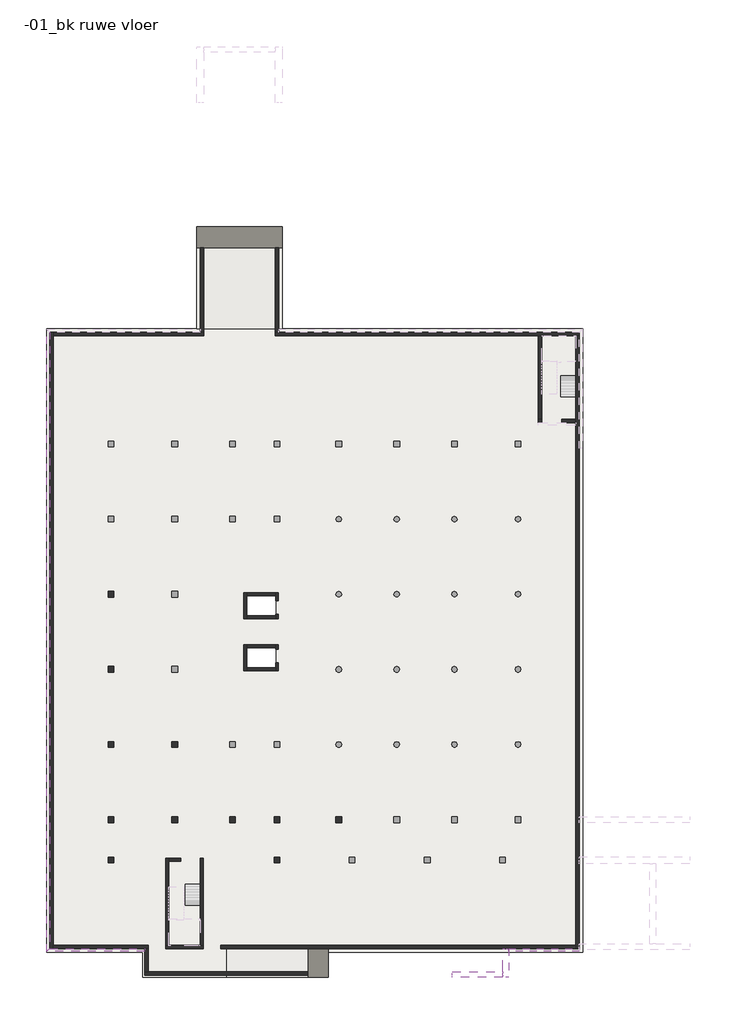
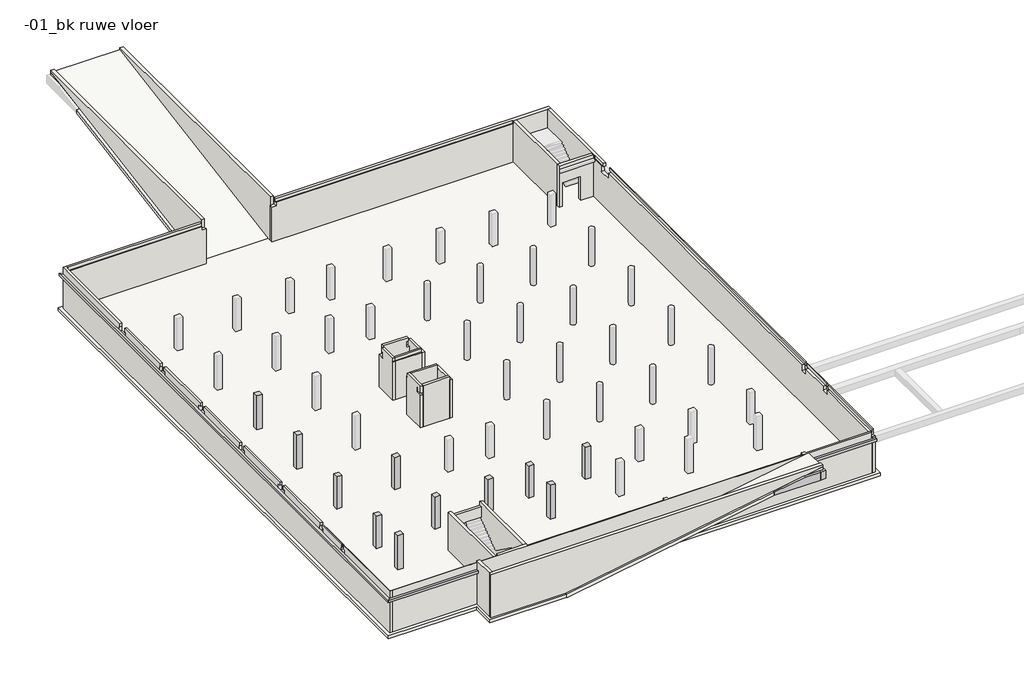
# One storey, part 1 of 2: 22 walls, 15 slabs, 11 columns, 5 beams.
# Revit data of these elements (continued)
# Grids (mm) (continued)
#   "L": line (13000, -4030.51) -> (13000, 79064.564)
# Type "NLRS_16_SF_LIB_oplegnok beton prefab framing-CWV-MMBPC-SRP_gen_rsf : oplegnok beton prefab_gen__bxh 250x250/220"
#   Export Type to IFC As = "IfcWallType"
#   Type IfcGUID = "2pBZpvCtn46PjCcATwz$Ih"
#   Type Comments = "oplegnok"
#   Model = "LOD300"
#   Description = "oplegnok beton prefab 250x250/220"
#   Assembly Code = "16.23"
#   NLRS_C_hoogte_01 = 220 mm
#   NLRS_C_hoogte = 250 mm
#   NLRS_C_breedte = 250 mm
#   Lossing = 30 mm
#   Length [instance default] = 3000 mm
#   Structural Material = NLRS_f2_beton prefab_gen_rsf
# Type "NLRS_16_SF_LIB_funderingsbalk beton ihwg-CWV-MMBC-SRP_gen_rsf : funderingsbalk beton ihwg_gen__bxh 500x800"
#   Export Type to IFC As = "IfcBeamType"
#   Type IfcGUID = "3yoae3mAzBRekDMiYpsxNi"
#   Type Comments = "500x800"
#   Model = "LOD300"
#   Description = "funderingsbalk beton ihwg 500x800"
#   Assembly Code = "16.12"
#   NLRS_C_lengte [instance default] = 3000 mm
#   NLRS_C_hoogte = 800 mm
#   NLRS_C_breedte = 500 mm
#   Length [instance default] = 3000 mm
#   Structural Material = NLRS_f2_beton ihwg_gen_rsf
# Type "NLRS_28_SCO_TLB_vierkante kolom beton prefab-BCPG-MMBPC-SRP_gen_rsf : kolom vierkant beton prefab_gen__bxh 500x500"
#   Type IFC Predefined Type = "COLUMN"
#   Export Type to IFC As = "IfcColumnType"
#   Type IfcGUID = "2bNskL0kfByRmbY5G6If6v"
#   Type Comments = "500x500"
#   Description = "prefab betonkolom 500x500"
#   Assembly Code = "28.11"
#   NLRS_C_lengte [instance default] = 2700 mm
#   NLRS_C_hoogte = 500 mm
#   NLRS_C_breedte = 500 mm
#   Structural Material = NLRS_f2_beton prefab_gen_rsf
#   Model = ""
# Type "NLRS_13_FL_beton ihwg 300_gen_rsf"
#   Keynote = ""
#   Export Type to IFC As = "IfcSlab"
#   Type IfcGUID = "2Gmsv2lRH0fOa54XIbCVVz"
#   Type Comments = "d=300mm"
#   Description = "300mm in het werk gestorte betonvloer"
#   Assembly Code = "13.22"
#   Function = 1
#   Layers, outside or top first: 300 mm "NLRS_f2_beton ihwg_gen_rsf" (function 1)
# Type "NLRS_16_SFO_LB_funderingspoer meerpaals beton ihwg-MMBC-SH_gen_rsf : funderingspoer beton ihwg_gen__4-paals bxlxh 1800x1800x1200"
#   Export Type to IFC As = "IfcFootingType"
#   Type IfcGUID = "0NibaB7BP2RgdAc9dAk106"
#   Type Comments = "4-paals poer 1800x1800x1200"
#   Model = " "
#   Manufacturer = " "
#   Keynote = "4-paals poer 1800x1800x1200"
#   Description = "4-paals poer 1800x1800x1200"
#   Assembly Code = "16.13"
#   Width = 1800 mm
#   Rough Height = 1200 mm
#   NLRS_C_lengte = 1800 mm
#   NLRS_C_hoogte = 1200 mm
#   NLRS_C_breedte = 1800 mm
#   Length = 1800 mm
#   Height [instance default] = 1050 mm
#   Foundation Thickness = 1200 mm
#   Depth [instance default] = 150 mm
#   Structural Material = NLRS_f2_beton ihwg_gen_rsf
# Type "NLRS_16_SFO_LB_funderingspoer meerpaals beton ihwg-MMBC-SH_gen_rsf : funderingspoer beton ihwg_gen__3-paals bxlxh 1800x1800x1200"
#   Export Type to IFC As = "IfcFootingType"
#   Type IfcGUID = "1GXoSzV6T12eGHLrhjoRUB"
#   Type Comments = "3-paals poer 1800x1800x1200"
#   Model = " "
#   Manufacturer = " "
#   Description = "3-paals poer 1800x1800x1200"
#   Assembly Code = "16.13"
#   Width = 1800 mm
#   Rough Height = 1200 mm
#   NLRS_C_lengte = 1800 mm
#   NLRS_C_hoogte = 1200 mm
#   NLRS_C_breedte = 1800 mm
#   Length = 1800 mm
#   Height [instance default] = 1050 mm
#   Foundation Thickness = 1200 mm
#   Depth [instance default] = 150 mm
#   Structural Material = NLRS_f2_beton ihwg_gen_rsf
#   Keynote = ""
# Type "NLRS_16_SFO_LB_funderingspoer meerpaals beton ihwg-MMBC-SH_gen_rsf : funderingspoer beton ihwg_gen__2-paals bxlxh 700x1800x1200"
#   Export Type to IFC As = "IfcFootingType"
#   Type IfcGUID = "1GXoSzV6T12eGHLrhjoRVK"
#   Type Comments = "2-paals poer 700x1800x1200"
#   Model = " "
#   Manufacturer = " "
#   Description = "2-paals poer 700x1800x1200"
#   Assembly Code = "16.13"
#   Width = 700 mm
#   Rough Height = 1200 mm
#   NLRS_C_lengte = 1800 mm
#   NLRS_C_hoogte = 1200 mm
#   NLRS_C_breedte = 700 mm
#   Length = 1800 mm
#   Height [instance default] = 1050 mm
#   Foundation Thickness = 1200 mm
#   Depth [instance default] = 150 mm
#   Structural Material = NLRS_f2_beton ihwg_gen_rsf
#   Keynote = ""
# Type "NLRS_16_SFO_LB_funderingspoer meerpaals beton ihwg-MMBC-SH_gen_rsf : funderingspoer beton ihwg_gen__1-paals bxlxh 700x700x500"
#   Export Type to IFC As = "IfcFootingType"
#   Type IfcGUID = "1GXoSzV6T12eGHLrhjoRTu"
#   Type Comments = "1-paals poer 700x700x500"
#   Model = " "
#   Manufacturer = " "
#   Description = "1-paals poer 700x700x500"
#   Assembly Code = "16.13"
#   Width = 700 mm
#   Rough Height = 500 mm
#   NLRS_C_lengte = 700 mm
#   NLRS_C_hoogte = 500 mm
#   NLRS_C_breedte = 700 mm
#   Length = 700 mm
#   Height [instance default] = 350 mm
#   Foundation Thickness = 500 mm
#   Depth [instance default] = 150 mm
#   Structural Material = NLRS_f2_beton ihwg_gen_rsf
#   Keynote = ""
# Type "NLRS_16_SFO_LB_funderingspoer meerpaals beton ihwg-MMBC-SH_gen_rsf : funderingspoer beton ihwg_gen__trap bxlxh 3800x9300x1200"
#   Export Type to IFC As = "IfcFootingType"
#   Type IfcGUID = "3Qemsd6Xj1WRJeMYmB12y4"
#   Type Comments = "trappenhuispoer 3800x9300x1200"
#   Model = " "
#   Manufacturer = " "
#   Keynote = "trappenhuispoer 3800x9300x1200"
#   Description = "trappenhuispoer 3800x9300x1200"
#   Assembly Code = "16.13"
#   Width = 3800 mm
#   Rough Height = 1200 mm
#   NLRS_C_lengte = 9300 mm
#   NLRS_C_hoogte = 1200 mm
#   NLRS_C_breedte = 3800 mm
#   Length = 9300 mm
#   Height [instance default] = 1050 mm
#   Foundation Thickness = 1200 mm
#   Depth [instance default] = 150 mm
#   Structural Material = NLRS_f2_beton ihwg_gen_rsf
# Type "NLRS_16_WA_hollewand 300_gen_rsf"
#   Keynote = ""
#   Export Type to IFC As = "IfcWall"
#   Type IfcGUID = "3S13A4zHzAqApml_3w1Yzy"
#   Description = "buitenwand holle wand, generiek"
#   Assembly Code = "16.23"
#   Layers, outside or top first: 60 mm "NLRS_f2_beton prefab_gen_rsf" (function 1); 0 mm "NLRS_f2_beton ihwg_gen_rsf" (function 1); 60 mm "NLRS_f2_beton prefab_gen_rsf" (function 1)
# Type "NLRS_16_WA_beton ihw 300_gen_rsf"
#   Keynote = ""
#   Export Type to IFC As = "IfcWall"
#   Type IfcGUID = "3S1HfGygHC08_ZXeiJ7DHR"
#   Description = "buitenwand beton ihw, generiek"
#   Assembly Code = "16.23"
#   Layers, outside or top first: 300 mm "NLRS_f2_beton ihwg_gen_rsf" (function 1)
# Type "NLRS_21_WA_beton ihw 250_gen_rsf"
#   Keynote = ""
#   Export Type to IFC As = "IfcWall"
#   Type IfcGUID = "1pBmRfcsbA7BE9s_rekBP3"
#   Description = "buitenwand beton ihw, generiek"
#   Assembly Code = "21.21"
#   Layers, outside or top first: 250 mm "NLRS_f2_beton ihwg_gen_rsf" (function 1)
# Type "NLRS_21_WA_beton prefab 300_gen_rsf"
#   Keynote = ""
#   Export Type to IFC As = "IfcWall"
#   Type IfcGUID = "2ajLwCSRTE_9I1Spg4sCru"
#   Description = "buitenwand beton prefab, generiek"
#   Assembly Code = "21.21"
#   Layers, outside or top first: 300 mm "NLRS_f2_beton prefab_gen_rsf" (function 1)
# Element 1 (IfcBeam, "NLRS_16_SF_LIB_oplegnok beton prefab framing-CWV-MMBPC-SRP_gen_rsf : oplegnok beton prefab_gen__bxh 250x250/220")
#   IfcGUID = "2xH6lYwJzDD8CTyoTIBXLI"
#   IsExternal = yes
#   LoadBearing = yes
#   Phase Created = NLRS_nieuw
#   Materials on its faces: "NLRS_f2_beton prefab_gen_rsf"
# Element 2 (IfcBeam, "NLRS_16_SF_LIB_oplegnok beton prefab framing-CWV-MMBPC-SRP_gen_rsf : oplegnok beton prefab_gen__bxh 250x250/220")
#   IfcGUID = "2xH6lYwJzDD8CTyoTIBXLo"
#   IsExternal = yes
#   LoadBearing = yes
#   Phase Created = NLRS_nieuw
#   Materials on its faces: "NLRS_f2_beton prefab_gen_rsf"
# Element 3 (IfcBeam, "NLRS_16_SF_LIB_funderingsbalk beton ihwg-CWV-MMBC-SRP_gen_rsf : funderingsbalk beton ihwg_gen__bxh 500x800")
#   IfcGUID = "3yoae3mAzBRekDMiYpswhz"
#   Comments = ""
#   NLRS_C_lengte = 2650 mm
#   IsExternal = yes
#   LoadBearing = yes
#   Phase Created = NLRS_nieuw
#   Materials on its faces: "NLRS_f2_beton ihwg_gen_rsf"
# Element 4 (IfcBeam, "NLRS_16_SF_LIB_funderingsbalk beton ihwg-CWV-MMBC-SRP_gen_rsf : funderingsbalk beton ihwg_gen__bxh 500x800")
#   IfcGUID = "3yoae3mAzBRekDMiYpswfN"
#   NLRS_C_lengte = 4866.131 mm
#   IsExternal = yes
#   LoadBearing = yes
#   Phase Created = NLRS_nieuw
#   Materials on its faces: "NLRS_f2_beton ihwg_gen_rsf"
# Element 5 (IfcBeam, "NLRS_16_SF_LIB_oplegnok beton prefab framing-CWV-MMBPC-SRP_gen_rsf : oplegnok beton prefab_gen__bxh 250x250/220")
#   IfcGUID = "3aMdMHoe12P9KDGPyaIhSi"
#   IsExternal = yes
#   LoadBearing = yes
#   Phase Created = NLRS_nieuw
#   Materials on its faces: "NLRS_f2_beton prefab_gen_rsf"
# Element 6 (IfcColumn, "NLRS_28_SCO_TLB_vierkante kolom beton prefab-BCPG-MMBPC-SRP_gen_rsf : kolom vierkant beton prefab_gen__bxh 500x500")
#   IfcGUID = "2bNskL0kfByRmbY5G6If5v"
#   IsExternal = yes
#   LoadBearing = yes
#   Phase Created = NLRS_nieuw
#   Materials on its faces: "NLRS_f2_beton prefab_gen_rsf"
# Element 7 (IfcColumn, "NLRS_28_SCO_TLB_vierkante kolom beton prefab-BCPG-MMBPC-SRP_gen_rsf : kolom vierkant beton prefab_gen__bxh 500x500")
#   IfcGUID = "2bNskL0kfByRmbY5G6If62"
#   IsExternal = yes
#   LoadBearing = yes
#   Phase Created = NLRS_nieuw
#   Materials on its faces: "NLRS_f2_beton prefab_gen_rsf"
# Element 8 (IfcColumn, "NLRS_28_SCO_TLB_vierkante kolom beton prefab-BCPG-MMBPC-SRP_gen_rsf : kolom vierkant beton prefab_gen__bxh 500x500")
#   IfcGUID = "2bNskL0kfByRmbY5G6If64"
#   IsExternal = yes
#   LoadBearing = yes
#   Phase Created = NLRS_nieuw
#   Materials on its faces: "NLRS_f2_beton prefab_gen_rsf"
# Element 9 (IfcColumn, "NLRS_28_SCO_TLB_vierkante kolom beton prefab-BCPG-MMBPC-SRP_gen_rsf : kolom vierkant beton prefab_gen__bxh 500x500")
#   IfcGUID = "2bNskL0kfByRmbY5G6If9_"
#   IsExternal = yes
#   LoadBearing = yes
#   Phase Created = NLRS_nieuw
#   Materials on its faces: "NLRS_f2_beton prefab_gen_rsf"
# Element 10 (IfcColumn, "NLRS_28_SCO_TLB_vierkante kolom beton prefab-BCPG-MMBPC-SRP_gen_rsf : kolom vierkant beton prefab_gen__bxh 500x500")
#   IfcGUID = "2fqjgN40rEBBKvfwcj0BX5"
#   IsExternal = yes
#   LoadBearing = yes
#   Phase Created = NLRS_nieuw
#   Materials on its faces: "NLRS_f2_beton prefab_gen_rsf"
# Element 11 (IfcColumn, "NLRS_28_SCO_TLB_vierkante kolom beton prefab-BCPG-MMBPC-SRP_gen_rsf : kolom vierkant beton prefab_gen__bxh 500x500")
#   IfcGUID = "2r1e$qonv1u8B8mI4Mnhtx"
#   IsExternal = yes
#   LoadBearing = yes
#   Phase Created = NLRS_nieuw
#   Materials on its faces: "NLRS_f2_beton prefab_gen_rsf"
# Element 12 (IfcColumn, "NLRS_28_SCO_TLB_vierkante kolom beton prefab-BCPG-MMBPC-SRP_gen_rsf : kolom vierkant beton prefab_gen__bxh 500x500")
#   IfcGUID = "2r1e$qonv1u8B8mI4Mnhtz"
#   IsExternal = yes
#   LoadBearing = yes
#   Phase Created = NLRS_nieuw
#   Materials on its faces: "NLRS_f2_beton prefab_gen_rsf"
# Element 13 (IfcColumn, "NLRS_28_SCO_TLB_vierkante kolom beton prefab-BCPG-MMBPC-SRP_gen_rsf : kolom vierkant beton prefab_gen__bxh 500x500")
#   IfcGUID = "2r1e$qonv1u8B8mI4Mnht$"
#   IsExternal = yes
#   LoadBearing = yes
#   Phase Created = NLRS_nieuw
#   Materials on its faces: "NLRS_f2_beton prefab_gen_rsf"
# Element 14 (IfcColumn, "NLRS_28_SCO_TLB_vierkante kolom beton prefab-BCPG-MMBPC-SRP_gen_rsf : kolom vierkant beton prefab_gen__bxh 500x500")
#   IfcGUID = "2r1e$qonv1u8B8mI4Mnhtn"
#   IsExternal = yes
#   LoadBearing = yes
#   Phase Created = NLRS_nieuw
#   Materials on its faces: "NLRS_f2_beton prefab_gen_rsf"
# Element 15 (IfcColumn, "NLRS_28_SCO_TLB_vierkante kolom beton prefab-BCPG-MMBPC-SRP_gen_rsf : kolom vierkant beton prefab_gen__bxh 500x500")
#   IfcGUID = "2r1e$qonv1u8B8mI4MnhnB"
#   IsExternal = yes
#   LoadBearing = yes
#   Phase Created = NLRS_nieuw
#   Materials on its faces: "NLRS_f2_beton prefab_gen_rsf"
# Element 16 (IfcColumn, "NLRS_28_SCO_TLB_vierkante kolom beton prefab-BCPG-MMBPC-SRP_gen_rsf : kolom vierkant beton prefab_gen__bxh 500x500")
#   IfcGUID = "3oP0NMpTfAUg2$4DiBSKtG"
#   IsExternal = yes
#   LoadBearing = yes
#   Phase Created = NLRS_nieuw
#   Materials on its faces: "NLRS_f2_beton prefab_gen_rsf"
# Element 17 (IfcSlab, "NLRS_13_FL_beton ihwg 300_gen_rsf")
#   IfcGUID = "2Gmsv2lRH0fOa54XIbCVVL"
#   Height Offset From Level = 0 mm
#   built-in parameter 1001954 = 1
#   IsExternal = yes
#   LoadBearing = yes
#   Phase Created = NLRS_nieuw
#   Materials on its faces: "NLRS_f2_beton ihwg_gen_rsf"
# Element 18 (IfcSlab, "NLRS_13_FL_beton ihwg 300_gen_rsf")
#   IfcGUID = "2Gmsv2lRH0fOa54XIbCUXg"
#   built-in parameter 1001955 = 3.14159 (stored number, unit not read)
#   Height Offset From Level = 0 mm
#   built-in parameter 1001954 = 1
#   IsExternal = yes
#   LoadBearing = yes
#   Phase Created = NLRS_nieuw
#   Materials on its faces: "NLRS_f2_beton ihwg_gen_rsf"
# Element 19 (IfcSlab, "NLRS_13_FL_beton ihwg 300_gen_rsf")
#   IfcGUID = "26lVpBsBf2MQJTQGM8Ms4Y"
#   Comments = ""
#   Height Offset From Level = 0 mm
#   built-in parameter 1001954 = 1
#   IsExternal = yes
#   LoadBearing = yes
#   Phase Created = NLRS_nieuw
#   Materials on its faces: "NLRS_f2_beton ihwg_gen_rsf"
# Element 20 (IfcSlab, "NLRS_16_SFO_LB_funderingspoer meerpaals beton ihwg-MMBC-SH_gen_rsf : funderingspoer beton ihwg_gen__4-paals bxlxh 1800x1800x1200")
#   IfcGUID = "1GXoSzV6T12eGHLrhjoRHH"
#   Height = 900 mm
#   Depth = 300 mm
#   IsExternal = yes
#   LoadBearing = yes
#   Phase Created = NLRS_nieuw
#   Materials on its faces: "NLRS_f2_beton ihwg_gen_rsf"
# Element 21 (IfcSlab, "NLRS_16_SFO_LB_funderingspoer meerpaals beton ihwg-MMBC-SH_gen_rsf : funderingspoer beton ihwg_gen__3-paals bxlxh 1800x1800x1200")
#   IfcGUID = "1GXoSzV6T12eGHLrhjoRH8"
#   Height = 900 mm
#   Depth = 300 mm
#   IsExternal = yes
#   LoadBearing = yes
#   Phase Created = NLRS_nieuw
#   Materials on its faces: "NLRS_f2_beton ihwg_gen_rsf"
# Element 22 (IfcSlab, "NLRS_16_SFO_LB_funderingspoer meerpaals beton ihwg-MMBC-SH_gen_rsf : funderingspoer beton ihwg_gen__2-paals bxlxh 700x1800x1200")
#   IfcGUID = "1GXoSzV6T12eGHLrhjoRHh"
#   Height = 900 mm
#   Depth = 300 mm
#   IsExternal = yes
#   LoadBearing = yes
#   Phase Created = NLRS_nieuw
#   Materials on its faces: "NLRS_f2_beton ihwg_gen_rsf"
# Element 23 (IfcSlab, "NLRS_16_SFO_LB_funderingspoer meerpaals beton ihwg-MMBC-SH_gen_rsf : funderingspoer beton ihwg_gen__2-paals bxlxh 700x1800x1200")
#   IfcGUID = "1GXoSzV6T12eGHLrhjoRVg"
#   Height = 900 mm
#   Depth = 300 mm
#   IsExternal = yes
#   LoadBearing = yes
#   Phase Created = NLRS_nieuw
#   Materials on its faces: "NLRS_f2_beton ihwg_gen_rsf"
# Element 24 (IfcSlab, "NLRS_16_SFO_LB_funderingspoer meerpaals beton ihwg-MMBC-SH_gen_rsf : funderingspoer beton ihwg_gen__2-paals bxlxh 700x1800x1200")
#   IfcGUID = "1GXoSzV6T12eGHLrhjoRST"
#   Height = 900 mm
#   Depth = 300 mm
#   IsExternal = yes
#   LoadBearing = yes
#   Phase Created = NLRS_nieuw
#   Materials on its faces: "NLRS_f2_beton ihwg_gen_rsf"
# Element 25 (IfcSlab, "NLRS_16_SFO_LB_funderingspoer meerpaals beton ihwg-MMBC-SH_gen_rsf : funderingspoer beton ihwg_gen__1-paals bxlxh 700x700x500")
#   IfcGUID = "1GXoSzV6T12eGHLrhjoRSM"
#   Height = 200 mm
#   Depth = 300 mm
#   IsExternal = yes
#   LoadBearing = yes
#   Phase Created = NLRS_nieuw
#   Materials on its faces: "NLRS_f2_beton ihwg_gen_rsf"
# Element 26 (IfcSlab, "NLRS_16_SFO_LB_funderingspoer meerpaals beton ihwg-MMBC-SH_gen_rsf : funderingspoer beton ihwg_gen__1-paals bxlxh 700x700x500")
#   IfcGUID = "1GXoSzV6T12eGHLrhjoRS9"
#   Height = 200 mm
#   Depth = 300 mm
#   IsExternal = yes
#   LoadBearing = yes
#   Phase Created = NLRS_nieuw
#   Materials on its faces: "NLRS_f2_beton ihwg_gen_rsf"
# Element 27 (IfcSlab, "NLRS_16_SFO_LB_funderingspoer meerpaals beton ihwg-MMBC-SH_gen_rsf : funderingspoer beton ihwg_gen__1-paals bxlxh 700x700x500")
#   IfcGUID = "1GXoSzV6T12eGHLrhjoRTF"
#   Height = 200 mm
#   Depth = 300 mm
#   IsExternal = yes
#   LoadBearing = yes
#   Phase Created = NLRS_nieuw
#   Materials on its faces: "NLRS_f2_beton ihwg_gen_rsf"
# Element 28 (IfcSlab, "NLRS_16_SFO_LB_funderingspoer meerpaals beton ihwg-MMBC-SH_gen_rsf : funderingspoer beton ihwg_gen__2-paals bxlxh 700x1800x1200")
#   IfcGUID = "3VXE8Tiz5F69n85q0kAzIM"
#   Height = 900 mm
#   Depth = 300 mm
#   IsExternal = yes
#   LoadBearing = yes
#   Phase Created = NLRS_nieuw
#   Materials on its faces: "NLRS_f2_beton ihwg_gen_rsf"
# Element 29 (IfcSlab, "NLRS_16_SFO_LB_funderingspoer meerpaals beton ihwg-MMBC-SH_gen_rsf : funderingspoer beton ihwg_gen__4-paals bxlxh 1800x1800x1200")
#   IfcGUID = "3Qemsd6Xj1WRJeMYmB12n_"
#   Height = 900 mm
#   Depth = 300 mm
#   IsExternal = yes
#   LoadBearing = yes
#   Phase Created = NLRS_nieuw
#   Materials on its faces: "NLRS_f2_beton ihwg_gen_rsf"
# Element 30 (IfcSlab, "NLRS_16_SFO_LB_funderingspoer meerpaals beton ihwg-MMBC-SH_gen_rsf : funderingspoer beton ihwg_gen__trap bxlxh 3800x9300x1200")
#   IfcGUID = "3Qemsd6Xj1WRJeMYmB12_u"
#   Height = 900 mm
#   Depth = 300 mm
#   IsExternal = yes
#   LoadBearing = yes
#   Phase Created = NLRS_nieuw
#   Materials on its faces: "NLRS_f2_beton ihwg_gen_rsf"
# Element 31 (IfcSlab, "NLRS_16_SFO_LB_funderingspoer meerpaals beton ihwg-MMBC-SH_gen_rsf : funderingspoer beton ihwg_gen__3-paals bxlxh 1800x1800x1200")
#   IfcGUID = "3loy75XKz2Rw4dS8JWiauh"
#   Height = 900 mm
#   Depth = 300 mm
#   IsExternal = yes
#   LoadBearing = yes
#   Phase Created = NLRS_nieuw
#   Materials on its faces: "NLRS_f2_beton ihwg_gen_rsf"
# Element 32 (IfcWall, "NLRS_16_WA_hollewand 300_gen_rsf")
#   IfcGUID = "3S13A4zHzAqApml_3w1Ywi"
#   Comments = ""
#   Top Offset = 0 mm
#   Base Offset = 0 mm
#   wall height = 4130 mm
#   IsExternal = yes
#   LoadBearing = yes
#   Phase Created = NLRS_nieuw
#   Base Constraint = -01_bk ruwe vloer
#   Top Constraint = 00_bk ruwe vloer
#   Materials on its faces: "NLRS_f2_beton_prefab_gen", "NLRS_f2_beton_ihwg_gen", "NLRS_f2_beton ihwg_gen_rsf"
# Element 33 (IfcWall, "NLRS_16_WA_hollewand 300_gen_rsf")
#   IfcGUID = "2QVj0Ej6XCV9jwcNWznZWx"
#   Comments = ""
#   Top Offset = 0 mm
#   Base Offset = 0 mm
#   wall height = 4130 mm
#   IsExternal = yes
#   LoadBearing = yes
#   Phase Created = NLRS_nieuw
#   Base Constraint = -01_bk ruwe vloer
#   Top Constraint = 00_bk ruwe vloer
#   Materials on its faces: "NLRS_f2_beton ihwg_gen_rsf", "NLRS_f2_beton_ihwg_gen"
# Element 34 (IfcWall, "NLRS_16_WA_hollewand 300_gen_rsf")
#   IfcGUID = "2QVj0Ej6XCV9jwcNWznZkF"
#   Comments = ""
#   Top Offset = 0 mm
#   Base Offset = 0 mm
#   wall height = 4130 mm
#   IsExternal = yes
#   LoadBearing = yes
#   Phase Created = NLRS_nieuw
#   Base Constraint = -01_bk ruwe vloer
#   Top Constraint = 00_bk ruwe vloer
#   Materials on its faces: "NLRS_f2_beton ihwg_gen_rsf", "NLRS_f2_beton_ihwg_gen"
# Element 35 (IfcWall, "NLRS_16_WA_hollewand 300_gen_rsf")
#   IfcGUID = "2QVj0Ej6XCV9jwcNWznZj0"
#   Comments = ""
#   Top Offset = 0 mm
#   Base Offset = 0 mm
#   wall height = 4130 mm
#   IsExternal = yes
#   LoadBearing = yes
#   Phase Created = NLRS_nieuw
#   Base Constraint = -01_bk ruwe vloer
#   Top Constraint = 00_bk ruwe vloer
#   Materials on its faces: "NLRS_f2_beton_prefab_gen", "NLRS_f2_beton ihwg_gen_rsf", "NLRS_f2_beton_ihwg_gen"
# Element 36 (IfcWall, "NLRS_16_WA_hollewand 300_gen_rsf")
#   IfcGUID = "2QVj0Ej6XCV9jwcNWznZhu"
#   Comments = ""
#   Top Offset = 0 mm
#   Base Offset = 0 mm
#   wall height = 4130 mm
#   IsExternal = yes
#   LoadBearing = yes
#   Phase Created = NLRS_nieuw
#   Base Constraint = -01_bk ruwe vloer
#   Top Constraint = 00_bk ruwe vloer
#   Materials on its faces: "NLRS_f2_beton ihwg_gen_rsf", "NLRS_f2_beton_ihwg_gen"
# Element 37 (IfcWall, "NLRS_16_WA_beton ihw 300_gen_rsf")
#   IfcGUID = "3S1HfGygHC08_ZXeiJ7DJS"
#   Comments = ""
#   Top Offset = 200 mm
#   Base Offset = 0 mm
#   wall height = 4330 mm
#   IsExternal = yes
#   LoadBearing = yes
#   Phase Created = NLRS_nieuw
#   Base Constraint = -01_bk ruwe vloer
#   Top Constraint = 00_bk ruwe vloer
#   Materials on its faces: "NLRS_f2_beton ihwg_gen_rsf"
# Element 38 (IfcWall, "NLRS_16_WA_beton ihw 300_gen_rsf")
#   IfcGUID = "3S1HfGygHC08_ZXeiJ7DCk"
#   Comments = ""
#   Top Offset = 200 mm
#   Base Offset = 0 mm
#   wall height = 4330 mm
#   IsExternal = yes
#   LoadBearing = yes
#   Phase Created = NLRS_nieuw
#   Base Constraint = -01_bk ruwe vloer
#   Top Constraint = 00_bk ruwe vloer
#   Materials on its faces: "NLRS_f2_beton ihwg_gen_rsf"
# Element 39 (IfcWall, "NLRS_21_WA_beton ihw 250_gen_rsf")
#   IfcGUID = "1pBmRfcsbA7BE9s_rekBNw"
#   Comments = ""
#   Top Offset = 0 mm
#   Base Offset = 0 mm
#   wall height = 3810 mm
#   IsExternal = yes
#   LoadBearing = yes
#   Phase Created = NLRS_nieuw
#   Base Constraint = -01_bk ruwe vloer
#   Top Constraint = 00_ok ruwe vloer
#   Materials on its faces: "NLRS_f2_beton ihwg_gen_rsf"
# Element 40 (IfcWall, "NLRS_21_WA_beton ihw 250_gen_rsf")
#   IfcGUID = "1pBmRfcsbA7BE9s_rekBQ8"
#   Comments = ""
#   Top Offset = 0 mm
#   Base Offset = 0 mm
#   wall height = 3810 mm
#   IsExternal = yes
#   LoadBearing = yes
#   Phase Created = NLRS_nieuw
#   Base Constraint = -01_bk ruwe vloer
#   Top Constraint = 00_ok ruwe vloer
#   Materials on its faces: "NLRS_f2_beton ihwg_gen_rsf"
# Element 41 (IfcWall, "NLRS_21_WA_beton ihw 250_gen_rsf")
#   IfcGUID = "1pBmRfcsbA7BE9s_rekBRV"
#   Top Offset = 0 mm
#   Base Offset = 0 mm
#   wall height = 4130 mm
#   IsExternal = yes
#   LoadBearing = yes
#   Phase Created = NLRS_nieuw
#   Base Constraint = -01_bk ruwe vloer
#   Top Constraint = 00_bk ruwe vloer
#   Materials on its faces: "NLRS_f2_beton ihwg_gen_rsf"
# Element 42 (IfcWall, "NLRS_21_WA_beton ihw 250_gen_rsf")
#   IfcGUID = "3iyfZByB98yevaQCZKiCIx"
#   Comments = ""
#   Top Offset = 0 mm
#   Base Offset = 0 mm
#   wall height = 4130 mm
#   IsExternal = yes
#   LoadBearing = yes
#   Phase Created = NLRS_nieuw
#   Base Constraint = -01_bk ruwe vloer
#   Top Constraint = 00_bk ruwe vloer
#   Materials on its faces: "NLRS_f2_beton ihwg_gen_rsf"
# Element 43 (IfcWall, "NLRS_21_WA_beton ihw 250_gen_rsf")
#   IfcGUID = "3iyfZByB98yevaQCZKiCGB"
#   Comments = ""
#   Top Offset = 0 mm
#   Base Offset = 0 mm
#   wall height = 4130 mm
#   IsExternal = yes
#   LoadBearing = yes
#   Phase Created = NLRS_nieuw
#   Base Constraint = -01_bk ruwe vloer
#   Top Constraint = 00_bk ruwe vloer
#   Materials on its faces: "NLRS_f2_beton ihwg_gen_rsf"
# Element 44 (IfcWall, "NLRS_21_WA_beton ihw 250_gen_rsf")
#   IfcGUID = "3iyfZByB98yevaQCZKiCGb"
#   Comments = ""
#   Top Offset = 0 mm
#   Base Offset = 0 mm
#   wall height = 4130 mm
#   IsExternal = yes
#   LoadBearing = yes
#   Phase Created = NLRS_nieuw
#   Base Constraint = -01_bk ruwe vloer
#   Top Constraint = 00_bk ruwe vloer
#   Materials on its faces: "NLRS_f2_beton ihwg_gen_rsf"
# Element 45 (IfcWall, "NLRS_21_WA_beton ihw 250_gen_rsf")
#   IfcGUID = "3iyfZByB98yevaQCZKiClS"
#   Comments = ""
#   Top Offset = 0 mm
#   Base Offset = 0 mm
#   wall height = 3810 mm
#   IsExternal = yes
#   LoadBearing = yes
#   Phase Created = NLRS_nieuw
#   Base Constraint = -01_bk ruwe vloer
#   Top Constraint = 00_ok ruwe vloer
#   Materials on its faces: "NLRS_f2_beton ihwg_gen_rsf"
# Element 46 (IfcWall, "NLRS_21_WA_beton ihw 250_gen_rsf")
#   IfcGUID = "3iyfZByB98yevaQCZKiCjh"
#   Comments = ""
#   Top Offset = 0 mm
#   Base Offset = 0 mm
#   wall height = 4130 mm
#   IsExternal = yes
#   LoadBearing = yes
#   Phase Created = NLRS_nieuw
#   Base Constraint = -01_bk ruwe vloer
#   Top Constraint = 00_bk ruwe vloer
#   Materials on its faces: "NLRS_f2_beton ihwg_gen_rsf"
# Element 47 (IfcWall, "NLRS_21_WA_beton ihw 250_gen_rsf")
#   IfcGUID = "3iyfZByB98yevaQCZKiCi9"
#   Comments = ""
#   Top Offset = 0 mm
#   Base Offset = 0 mm
#   wall height = 4130 mm
#   IsExternal = yes
#   LoadBearing = yes
#   Phase Created = NLRS_nieuw
#   Base Constraint = -01_bk ruwe vloer
#   Top Constraint = 00_bk ruwe vloer
#   Materials on its faces: "NLRS_f2_beton ihwg_gen_rsf"
# Element 48 (IfcWall, "NLRS_21_WA_beton ihw 250_gen_rsf")
#   IfcGUID = "3iyfZByB98yevaQCZKiCik"
#   Comments = ""
#   Top Offset = 0 mm
#   Base Offset = 0 mm
#   wall height = 4130 mm
#   IsExternal = yes
#   LoadBearing = yes
#   Phase Created = NLRS_nieuw
#   Base Constraint = -01_bk ruwe vloer
#   Top Constraint = 00_bk ruwe vloer
#   Materials on its faces: "NLRS_f2_beton ihwg_gen_rsf"
# Element 49 (IfcWall, "NLRS_21_WA_beton prefab 300_gen_rsf")
#   IfcGUID = "2ajLwCSRTE_9I1Spg4sCjz"
#   Comments = ""
#   built-in parameter 1001111 = 30 mm
#   Top Offset = 0 mm
#   Base Offset = 30 mm
#   wall height = 4100 mm
#   IsExternal = yes
#   LoadBearing = yes
#   Phase Created = NLRS_nieuw
#   Base Constraint = -01_bk ruwe vloer
#   Top Constraint = 00_bk ruwe vloer
#   Materials on its faces: "NLRS_f2_beton prefab_gen_rsf"
# Element 50 (IfcWall, "NLRS_21_WA_beton prefab 300_gen_rsf")
#   IfcGUID = "2ajLwCSRTE_9I1Spg4sCjn"
#   Comments = ""
#   built-in parameter 1001111 = 30 mm
#   Top Offset = 0 mm
#   Base Offset = 30 mm
#   wall height = 4100 mm
#   IsExternal = yes
#   LoadBearing = yes
#   Phase Created = NLRS_nieuw
#   Base Constraint = -01_bk ruwe vloer
#   Top Constraint = 00_bk ruwe vloer
#   Materials on its faces: "NLRS_f2_beton prefab_gen_rsf"
# Element 51 (IfcWall, "NLRS_21_WA_beton ihw 250_gen_rsf")
#   IfcGUID = "1YBZRJosH5dOaCCgeRHuc1"
#   Comments = ""
#   Top Offset = 0 mm
#   Base Offset = 0 mm
#   wall height = 3810 mm
#   IsExternal = yes
#   LoadBearing = yes
#   Phase Created = NLRS_nieuw
#   Base Constraint = -01_bk ruwe vloer
#   Top Constraint = 00_ok ruwe vloer
#   Materials on its faces: "NLRS_f2_beton ihwg_gen_rsf"
# Element 52 (IfcWall, "NLRS_16_WA_beton ihw 300_gen_rsf")
#   IfcGUID = "26lVpBsBf2MQJTQGM8MsEk"
#   Comments = ""
#   Top Offset = 200 mm
#   Base Offset = 0 mm
#   wall height = 4330 mm
#   IsExternal = yes
#   LoadBearing = yes
#   Phase Created = NLRS_nieuw
#   Base Constraint = -01_bk ruwe vloer
#   Top Constraint = 00_bk ruwe vloer
#   Materials on its faces: "NLRS_f2_beton ihwg_gen_rsf"
# Element 53 (IfcWall, "NLRS_16_WA_beton ihw 300_gen_rsf")
#   IfcGUID = "26lVpBsBf2MQJTQGM8MsE9"
#   Comments = ""
#   Top Offset = 200 mm
#   Base Offset = 0 mm
#   wall height = 4330 mm
#   IsExternal = yes
#   LoadBearing = yes
#   Phase Created = NLRS_nieuw
#   Base Constraint = -01_bk ruwe vloer
#   Top Constraint = 00_bk ruwe vloer
#   Materials on its faces: "NLRS_f2_beton ihwg_gen_rsf"
# Materials
#   "NLRS_f2_beton prefab_gen_rsf": class "F - Niet gebakken kunststeen", colour RGB 129 133 118, transparency 0, Keynote = "f2", Manufacturer = "Revit Standards Foundation", URL = "www.revitstandards.org", Description = "beton prefab", Cost = 0
#   "NLRS_f2_beton ihwg_gen_rsf": class "F - Niet gebakken kunststeen", colour RGB 129 133 118, transparency 0, Keynote = "f2", Manufacturer = "Revit Standards Foundation", URL = "www.revitstandards.org", Description = "beton ihwg", Cost = 0
#   "NLRS_f2_beton_prefab_gen": class "Concrete", colour RGB 114 115 106, transparency 0, Manufacturer = "RevitGG", URL = "www.revitgg.nl", Description = "Beton, geprefabriceerd, generiek materiaal", Cost = 0
#   "NLRS_f2_beton_ihwg_gen": class "Concrete", colour RGB 192 192 192, transparency 0, Manufacturer = "RevitGG", URL = "www.revitgg.nl", Description = "Beton, generiek materiaal", Cost = 0
